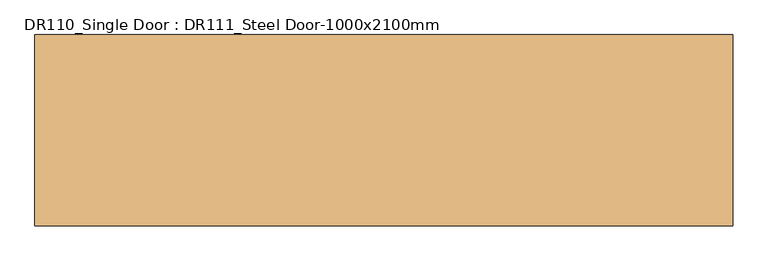
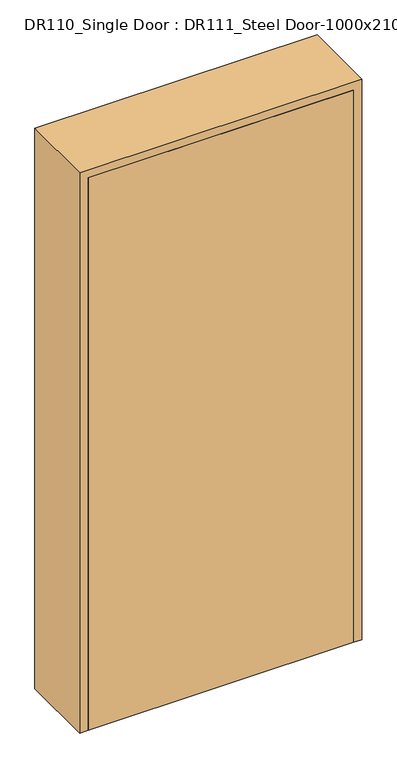
"""IFC4 building model written with IfcOpenShell, lengths in millimetres: door geometry, DR110_Single Door : DR111_Steel Door-1000x2100mm."""

from ifc_helpers import new_model, si_unit, origin, origin_with_axes, place, context, project, spatial, polyline, outline, extrude, faceted_brep, source, transform, mapped, element, save


def dr110_single_door_dr111_steel_door_1000x2100mm_c730d40a(model_context):
    return source(origin(), model_context, "Body", "SolidModel", [
        extrude(outline(polyline([(470.0, -137.0), (-470.0, -137.0), (-470.0, -102.0), (470.0, -102.0), (470.0, -137.0)])), origin_with_axes(), (0.0, 0.0, 1.0), 2070.0),
        faceted_brep([(470.0, -137.0, 0.0), (470.0, -102.0, 0.0), (450.0, -102.0, 0.0), (450.0, 102.0, 0.0), (470.0, 102.0, 0.0), (470.0, 137.0, 0.0), (500.0, 137.0, 0.0), (500.0, -137.0, 0.0), (500.0, -137.0, 2100.0), (-500.0, -137.0, 2100.0), (-500.0, -137.0, 0.0), (-470.0, -137.0, 0.0), (-470.0, -137.0, 2070.0), (470.0, -137.0, 2070.0), (500.0, 137.0, 2100.0), (470.0, 137.0, 2070.0), (-470.0, 137.0, 2070.0), (-470.0, 137.0, 0.0), (-500.0, 137.0, 0.0), (-500.0, 137.0, 2100.0), (470.0, 102.0, 2070.0), (450.0, 102.0, 2050.0), (-450.0, 102.0, 2050.0), (-450.0, 102.0, 0.0), (-470.0, 102.0, 0.0), (-470.0, 102.0, 2070.0), (450.0, -102.0, 2050.0), (470.0, -102.0, 2070.0), (-470.0, -102.0, 2070.0), (-470.0, -102.0, 0.0), (-450.0, -102.0, 0.0), (-450.0, -102.0, 2050.0)], [[[0, 1, 2, 3, 4, 5, 6, 7]], [[7, 8, 9, 10, 11, 12, 13, 0]], [[6, 14, 8, 7]], [[5, 15, 16, 17, 18, 19, 14, 6]], [[4, 20, 15, 5]], [[3, 21, 22, 23, 24, 25, 20, 4]], [[2, 26, 21, 3]], [[1, 27, 28, 29, 30, 31, 26, 2]], [[0, 13, 27, 1]], [[12, 11, 29, 28]], [[11, 10, 18, 17, 24, 23, 30, 29]], [[19, 18, 10, 9]], [[25, 24, 17, 16]], [[31, 30, 23, 22]], [[14, 19, 9, 8]], [[20, 25, 16, 15]], [[26, 31, 22, 21]], [[13, 12, 28, 27]]]),
    ])


if __name__ == "__main__":
    model = new_model("IFC4")
    model_context = context("Model", 3, world=origin())
    ifc_project = project(units=[si_unit("LENGTHUNIT", "METRE", prefix="MILLI")], contexts=[model_context])
    site = spatial("IfcSite", under=ifc_project)
    building = spatial("IfcBuilding", under=site)
    placement = place(None, origin())
    dr110_single_door_dr111_steel_door_1000x2100mm_shape = dr110_single_door_dr111_steel_door_1000x2100mm_c730d40a(model_context)
    element("IfcDoor", 1, ObjectType="DR110_Single Door : DR111_Steel Door-1000x2100mm", at=placement, inside=building, context=model_context, shape_type="MappedRepresentation", body=[
        mapped(dr110_single_door_dr111_steel_door_1000x2100mm_shape, transform((0.0, 0.0, 0.0), x_axis=(1.0, 0.0, 0.0), y_axis=(0.0, 1.0, 0.0), z_axis=(0.0, 0.0, 1.0))),
    ])
    save(model, "model.ifc")

# Revit data of these elements
# Type "DR110_Single Door : DR111_Steel Door-1000x2100mm"
#   Type Mark = "SD"
#   Analytic Construction = "<None>"
#   프레임 투영 외부. = 25 mm
#   프레임 투영 내부. = 25 mm
#   프레임 폭 = 75 mm
#   Height = 2100 mm
#   Width = 1000 mm
#   Define Thermal Properties by = 1
#   문 패널 = SD1 문 패널
#   문 프레임 = A04AQ098-00002_Steel Door_non FP_single
#   Function = (empty or 0)
#   Wall Closure = (empty or 0)
# Element 1 (IfcDoor, "DR110_Single Door : DR111_Steel Door-1000x2100mm")
#   Materials on its faces: "A04AQ098-00002_Steel Door_non FP_single", "SD1 문 패널"
# Materials
#   "SD1 문 패널": class "금속", colour RGB 247 247 247, transparency 0, Description = "STEEL DOOR (1000Wx2100H)"
#   "A04AQ098-00002_Steel Door_non FP_single": class "금속", colour RGB 247 247 247, transparency 0, Description = "Steel Door", W00) Work Master Code = "A04AQ098-00002", W01) Work Master_Lv1 = "Finishing Work", W02) Work Master_Lv2 = "Door & Window Work", W03) Work Master_Spec.1 = "Steel Door w/ Steel Frame", W04) Work Master_Spec.2 = "Fire Protective Rating: N/A, Single Door", W05) Work Master_Spec.3 = "w/ Hardware & Accessories", Cost = 0
